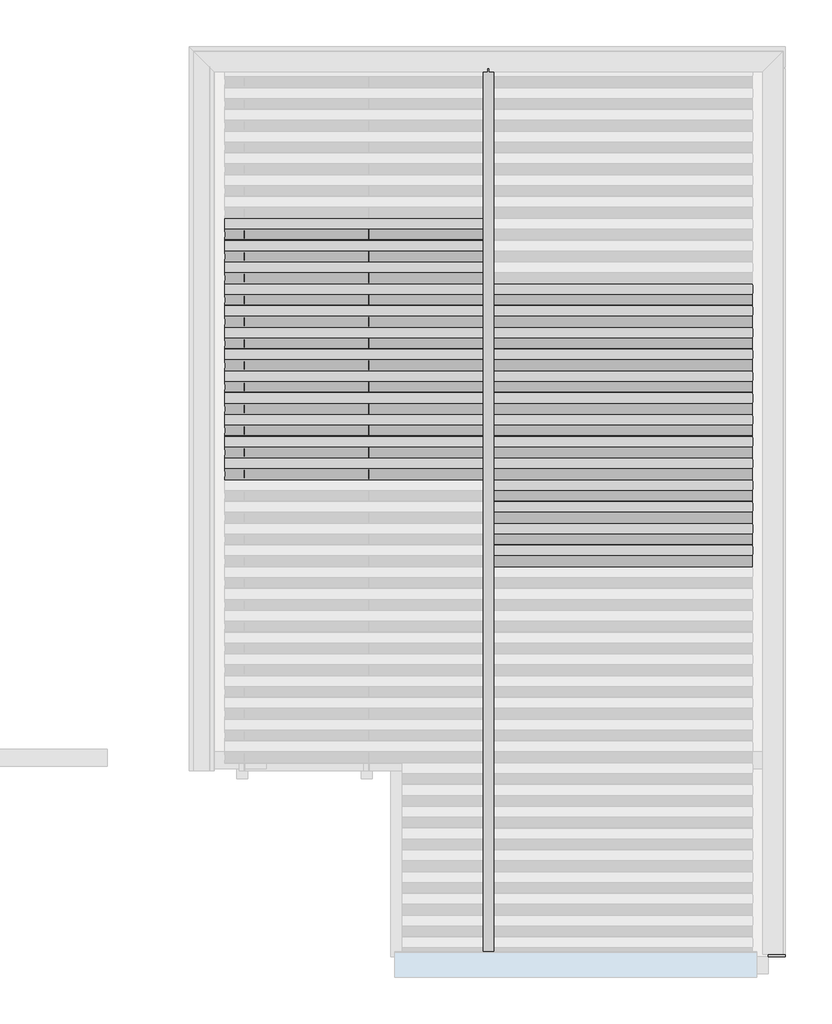
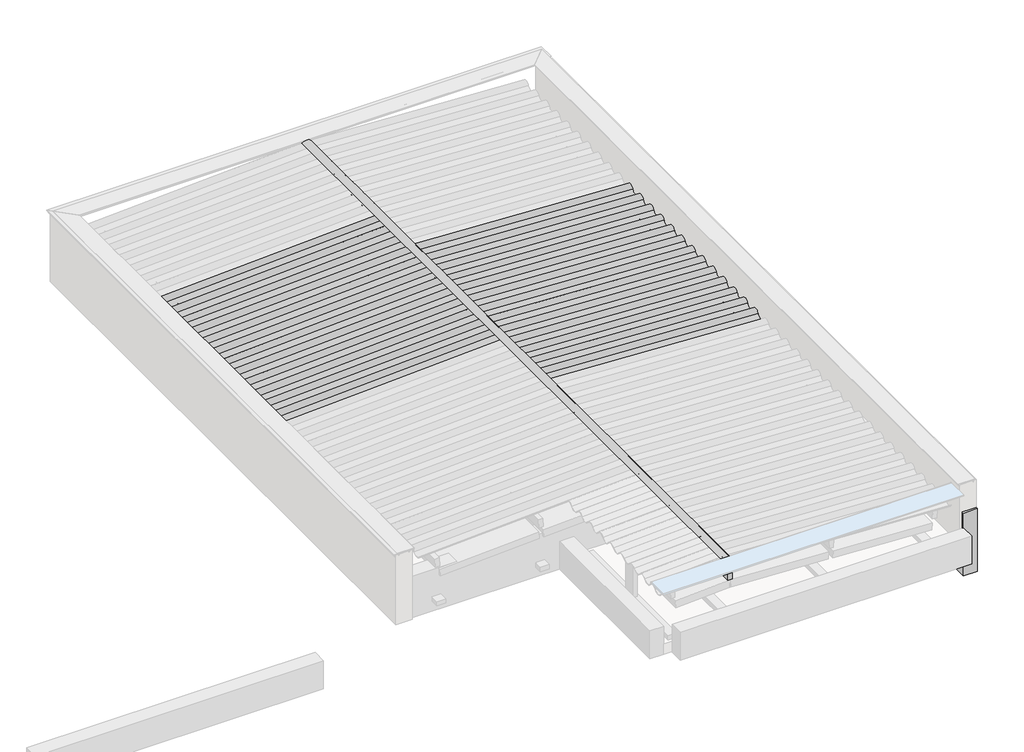
# One storey, part 3 of 4: 37 beams, 8 columns.
# Revit data of these elements (continued)
# Element 11 (IfcBeam, "TQS - Viga retangular : 19.0 x 90.0") (continued)
#   Tipo de carga = ""
#   Divisor de flexao = ""
#   Secao = ""
#   Configuracao = ""
#   Angulo (graus) = ""
#   Detalhamento = ""
#   Casos de vento manual = ""
#   Tipo = ""
#   Alcas = ""
#   Furos = ""
#   Pino = ""
#   Distribuicao = ""
#   Solidarizado = ""
#   Solidarizar na montagem = ""
#   Unir com o próximo = ""
#   Grupo pre moldado = ""
#   Verificado = ""
#   Concreto C = ""
#   Taxa de armadura (kgf/m³) = 0
#   Carga (tf/m²) = 0
#   Carga (tf/m) = 0
#   Carga (tf) = 0
#   Altura = 0.90 m
#   Rebaixo = -0.45 m
#   Largura = 0.19 m
#   Distancia a face = 0.00 m
#   Distancia ao eixo = 0.00 m
#   Altura gerber esquerda = 0.00 m
#   Largura gerber esquerda = 0.00 m
#   Altura gerber direita = 0.00 m
#   Largura gerber direita = 0.00 m
#   Resultado de Ensaios fck (MPa) = 0
#   Unique TQS ID = -298
#   Principal = yes
#   Structural Material = none
#   Phase Created = CC_PE
# Elements 12, 13, 14, 15, 16, 17, 18, 19, 20, 21, 22, 23, 24, 25, 26, 27, 28, 29, 30, 31, 32, 33, 34, 35, 36 (IfcBeam, "Telha Ondulada : Fibrocimento")
#   Phase Created = CC_PE
#   Materials on its faces: ".TELHA DE FIBROCIMENTO"
# Element 37 (IfcBeam, "Madeira de lei : Viga Cumeeira 6x16cm")
#   Comments = ""
#   Structural Material = .MADEIRAMENTO
#   Phase Created = CC_PE
#   Materials on its faces: ".MADEIRAMENTO"
# Elements 38, 39, 40, 41, 42, 43, 44, 45 (IfcColumn, "Madeira de lei-Coluna : Pontalete 6X16cm")
#   Comments = ""
#   Structural Material = .MADEIRAMENTO
#   Phase Created = CC_PE
#   Materials on its faces: ".MADEIRAMENTO"
# Materials
#   ".TELHA DE FIBROCIMENTO": class "CC_TELHADO", colour RGB 77 77 76, transparency 0, Description = "TELHA ONDULADA FIBROCIMENTO", Cost = 0
#   ".MADEIRAMENTO": class ".CC_MADEIRAS", colour RGB 212 179 113, transparency 0, Cost = 0
